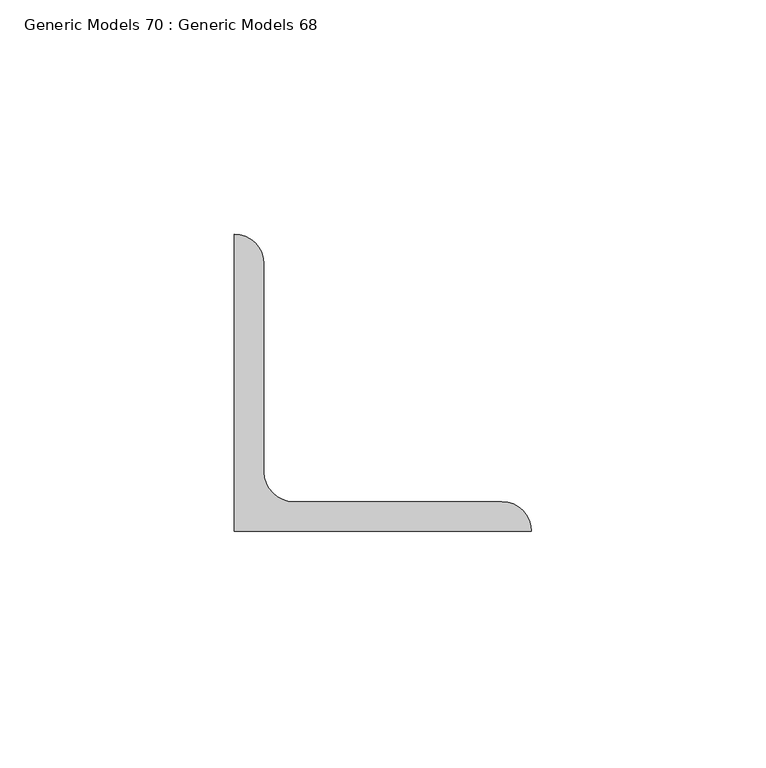
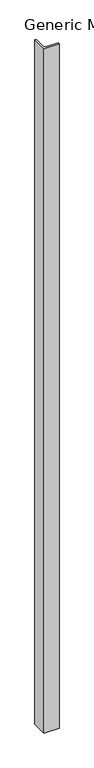
"""IFC4 building model written with IfcOpenShell, lengths in millimetres: proxy geometry, Generic Models 70 : Generic Models 68."""

from ifc_helpers import new_model, si_unit, point, frame, frame_2d, origin, place, context, project, spatial, polyline, circle_curve, trimmed, segment, composite_curve, outline, extrude, source, transform, mapped, element, save


def generic_models_70_generic_models_68_6c993f07(model_context):
    return source(origin(), model_context, "Body", "SweptSolid", [
        extrude(outline(composite_curve([segment(polyline([(20530.4116945, 18496.0264581), (20530.4116945, 18559.5264581)]), True, "CONTINUOUS"), segment(trimmed(circle_curve(frame_2d((20530.4116945, 18553.1764581)), 6.35), [point((20530.4116945, 18559.5264581))], [point((20536.7616945, 18553.1764581))], False, "CARTESIAN"), True, "CONTINUOUS"), segment(polyline([(20536.7616945, 18553.1764581), (20536.7616945, 18508.7264581)]), True, "CONTINUOUS"), segment(trimmed(circle_curve(frame_2d((20543.1116945, 18508.7264581)), 6.35), [point((20536.7616945, 18508.7264581))], [point((20543.1116945, 18502.3764581))], True, "CARTESIAN"), True, "CONTINUOUS"), segment(polyline([(20543.1116945, 18502.3764581), (20587.5616945, 18502.3764581)]), True, "CONTINUOUS"), segment(trimmed(circle_curve(frame_2d((20587.5616945, 18496.0264581)), 6.35), [point((20587.5616945, 18502.3764581))], [point((20593.9116945, 18496.0264581))], False, "CARTESIAN"), True, "CONTINUOUS"), segment(polyline([(20593.9116945, 18496.0264581), (20530.4116945, 18496.0264581)]), True, "CONTINUOUS")], self_intersect=False)), frame((0.0, 0.0, 264380.6186948), z_axis=(0.0, 0.0, 1.0), x_axis=(1.0, 0.0, 0.0)), (0.0, 0.0, 1.0), 3006.09),
    ])


if __name__ == "__main__":
    model = new_model("IFC4")
    model_context = context("Model", 3, world=origin())
    ifc_project = project(units=[si_unit("LENGTHUNIT", "METRE", prefix="MILLI")], contexts=[model_context])
    site = spatial("IfcSite", under=ifc_project)
    building = spatial("IfcBuilding", under=site)
    placement = place(None, origin())
    generic_models_70_generic_models_68_shape = generic_models_70_generic_models_68_6c993f07(model_context)
    element("IfcBuildingElementProxy", 1, Name="Generic Models 70 : Generic Models 68", ObjectType="Generic Models 70 : Generic Models 68", at=placement, inside=building, context=model_context, shape_type="MappedRepresentation", body=[
        mapped(generic_models_70_generic_models_68_shape, transform((0.0, 0.0, 0.0), x_axis=(1.0, 0.0, 0.0), y_axis=(0.0, 1.0, 0.0), z_axis=(0.0, 0.0, 1.0))),
    ])
    save(model, "model.ifc")

# Revit data of these elements
# Element 1 (IfcBuildingElementProxy, "Generic Models 70 : Generic Models 68")
#   Materials on its faces: "MAIN FENCE POST: (2) BACK/BACK GALVANIZED ANGLES (2) L2 1/2 X 2 1/2 X 1/4\") ANCHORED TO 8\"W X 42\" DEEP CONCRETE FOOTING(1)"
# Materials
#   "MAIN FENCE POST: (2) BACK/BACK GALVANIZED ANGLES (2) L2 1/2 X 2 1/2 X 1/4\") ANCHORED TO 8\"W X 42\" DEEP CONCRETE FOOTING(1)": class "Unassigned", colour RGB 211 211 211, transparency 0, Cost = 0
